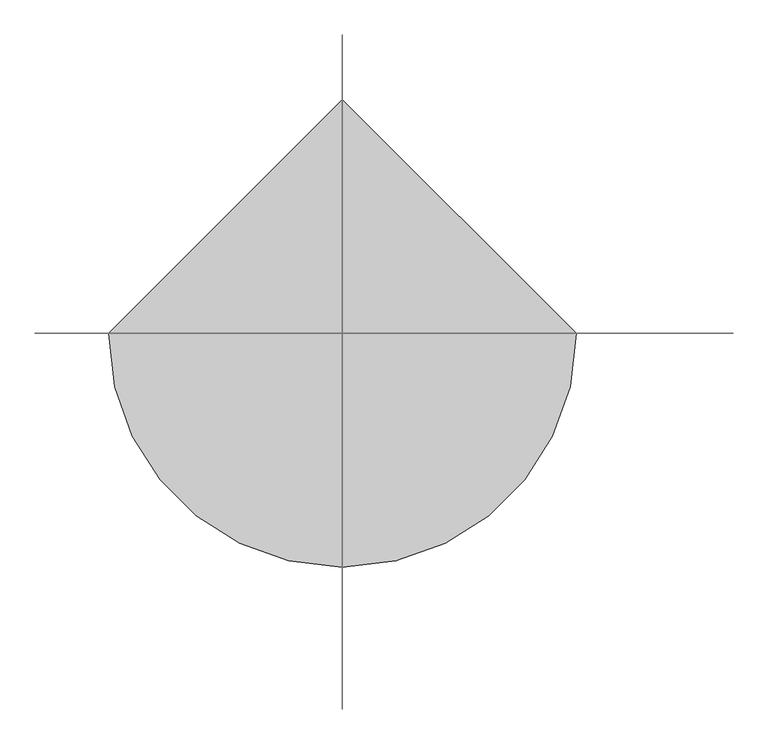
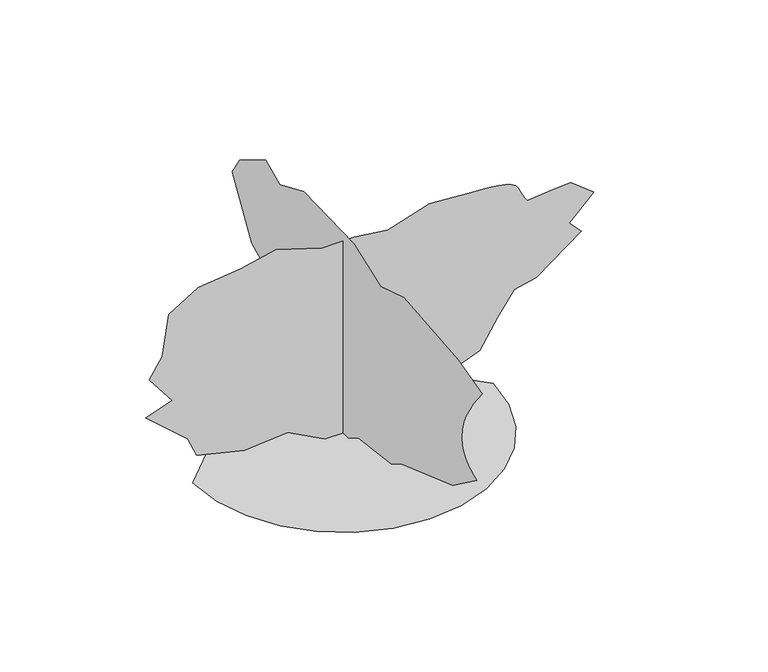
"""IFC4 building model written with IfcOpenShell, lengths in millimetres: proxy geometry, meyer lilac 26082 : meyer lilac 26082."""

from ifc_helpers import new_model, si_unit, origin, place, context, project, spatial, triangles, source, transform, mapped, element, save


def entourage_ea84321d(model_context):
    return source(origin(), model_context, "Body", "Tessellation", [
        triangles([(-84.8149175, 7.75e-05, 8.6e-06), (-258.4957951, 7.39e-05, 93.6967881), (-462.1199759, 8.49e-05, 75.7298434), (-683.7121187, 8.82e-05, 129.6306776), (-725.6373213, 7.86e-05, 225.4544616), (-923.2722055, 6.65e-05, 399.1355936), (-797.5040829, 5.6e-05, 441.0582891), (-905.306805, 4.43e-05, 578.805041), (-845.4161293, 3.03e-05, 674.6290976), (-815.4720268, 5.4e-06, 872.2639091), (-677.7253475, -1.06e-05, 956.1093), (-480.0879198, -2.21e-05, 980.0666313), (-312.397138, -3.37e-05, 1015.9999758), (-96.7927928, -3.53e-05, 950.1199854), (52.9315665, -4.18e-05, 950.1199854), (208.6452405, -4.65e-05, 932.1545849), (406.2806153, -6.23e-05, 992.0452606), (615.896636, -7e-05, 980.0666313), (655.4622442, -7.14e-05, 977.3944834), (693.7171766, -7.27e-05, 974.0950481), (729.355917, -7.37e-05, 969.5382769), (761.0627026, -7.43e-05, 963.0943388), (787.5346333, -7.44e-05, 954.1382721), (807.455801, -7.38e-05, 942.0377026), (819.5208349, -7.25e-05, 926.1652702), (826.871549, -7.08e-05, 909.594334), (833.5949759, -6.94e-05, 895.540468), (839.7925627, -6.83e-05, 883.5796429), (845.5736052, -6.73e-05, 873.2951689), (851.0371525, -6.65e-05, 864.2680309), (856.2924276, -6.57e-05, 856.0790686), (861.443494, -6.5e-05, 848.309194), (975.2355309, -7.14e-05, 860.2852798), (1065.0702364, -7.61e-05, 866.2745945), (1172.8703424, -7.08e-05, 782.4292036), (1059.0809217, -5.23e-05, 668.6397102), (1112.9822828, -4.75e-05, 608.7490708), (903.3662258, -1.97e-05, 453.0343749), (801.5554344, -1.24e-05, 429.0796597), (723.6968147, 3.8e-06, 321.2769739), (639.8513512, 2.39e-05, 183.5315118), (328.4245391, 5.18e-05, 63.7517137), (202.6561802, 5.51e-05, 81.7186584), (100.8435812, 6.93e-05, 5e-07), (0.021362, 58.648346, 1.19e-05), (0.0213578, 202.8161995, 40.9414963), (0.021352, 346.9843074, 46.4863159), (0.021347, 407.9773141, 151.839669), (0.0213581, 335.8946863, 196.1989981), (0.0213523, 457.8832432, 223.9235958), (0.0213509, 607.5959435, 323.7331467), (0.0213526, 563.2348432, 406.9054682), (0.0213517, 740.6741215, 490.0802968), (0.0213453, 895.9316505, 750.6918966), (0.021359, 834.9361004, 844.9538755), (0.0213677, 624.230357, 972.4872248), (0.0213728, 513.3314575, 917.0390104), (0.0213802, 319.2602002, 1000.2113319), (0.0213989, -85.5197618, 989.1216745), (0.0214104, -307.3171429, 911.4942181), (0.0214172, -490.2987428, 966.9424324), (0.021433, -933.8919062, 928.1286678), (0.0214469, -1127.9631998, 878.2227751), (0.0214342, -1091.3973358, 830.7450771), (0.0214336, -1056.4291214, 783.5569691), (0.021433, -1024.6639091, 736.9505116), (0.0214322, -997.699276, 691.2152945), (0.0214311, -977.1354149, 646.6458492), (0.0214298, -964.575135, 603.5319111), (0.0214281, -961.6160133, 562.1629609), (0.0214263, -967.0643726, 525.9679318), (0.0214245, -978.0421909, 497.337085), (0.0214229, -993.625106, 475.0130116), (0.0214213, -1012.893552, 457.7308542), (0.0214197, -1034.9280355, 444.2332769), (0.0214305, -1058.8065926, 433.2554223), (0.021429, -1083.6046429, 423.5399179), (0.0214189, -889.5333492, 279.3720463), (0.0213939, -473.6642567, 135.2049558), (0.021383, -390.489428, 85.3005619), (0.0213686, -124.3337626, 52.0311355), (0.0213699, -41.160192, 0.0), (-701.8553427, 0.0, 8.48e-05), (-683.3005886, -160.8188175, 0.000114), (-630.4584652, -308.5058421, 9.41e-05), (-547.5554223, -438.8281563, 0.0001242), (-438.8281563, -547.5554223, 0.0001065), (-308.5058421, -630.4559217, 9.09e-05), (-160.8188175, -683.3005886, 0.0001273), (3.04e-05, -701.8553427, 0.0001181), (160.8190719, -683.3005886, 0.0001133), (308.5058421, -630.4559217, 0.0001131), (438.8281563, -547.5554223, 0.0001173), (547.5554223, -438.8281563, 0.0001255), (630.4559217, -308.5058421, 8.82e-05), (683.3005886, -160.8188175, 0.0001035), (701.8553427, 6.14e-05, 0.0001219), (-9.28e-05, 701.8553427, 8.86e-05)], [[5, 6, 7], [34, 35, 36], [33, 34, 36], [36, 37, 38], [32, 33, 36], [32, 36, 38], [32, 38, 39], [7, 8, 9], [3, 4, 5], [9, 10, 11], [9, 11, 12], [7, 9, 12], [5, 7, 12], [3, 5, 12], [2, 3, 12], [2, 12, 13], [2, 13, 14], [2, 14, 15], [1, 2, 15], [44, 1, 15], [43, 44, 15], [43, 15, 16], [42, 43, 16], [41, 42, 16], [40, 41, 16], [40, 16, 17], [39, 40, 17], [32, 39, 17], [32, 17, 18], [32, 18, 19], [31, 32, 19], [30, 31, 19], [30, 19, 20], [29, 30, 20], [29, 20, 21], [28, 29, 21], [27, 28, 21], [27, 21, 22], [26, 27, 22], [26, 22, 23], [26, 23, 24], [26, 24, 25], [76, 77, 78], [62, 63, 64], [75, 76, 78], [74, 75, 78], [62, 64, 65], [47, 48, 49], [46, 47, 49], [50, 51, 52], [73, 74, 78], [62, 65, 66], [53, 54, 55], [53, 55, 56], [53, 56, 57], [52, 53, 57], [72, 73, 78], [52, 57, 58], [52, 58, 59], [50, 52, 59], [49, 50, 59], [49, 59, 60], [46, 49, 60], [45, 46, 60], [82, 45, 60], [81, 82, 60], [80, 81, 60], [79, 80, 60], [78, 79, 60], [78, 60, 61], [72, 78, 61], [71, 72, 61], [70, 71, 61], [70, 61, 62], [69, 70, 62], [68, 69, 62], [67, 68, 62], [67, 62, 66], [97, 98, 83], [96, 97, 83], [96, 83, 84], [95, 96, 84], [95, 84, 85], [95, 85, 86], [94, 95, 86], [93, 94, 86], [93, 86, 87], [93, 87, 88], [93, 88, 89], [93, 89, 90], [93, 90, 91], [93, 91, 92]], closed=False),
    ])


if __name__ == "__main__":
    model = new_model("IFC4")
    model_context = context("Model", 3, world=origin())
    ifc_project = project(units=[si_unit("LENGTHUNIT", "METRE", prefix="MILLI")], contexts=[model_context])
    site = spatial("IfcSite", under=ifc_project)
    building = spatial("IfcBuilding", under=site)
    placement = place(None, origin())
    entourage_shape = entourage_ea84321d(model_context)
    element("IfcBuildingElementProxy", 1, Name="meyer lilac 26082 : meyer lilac 26082", ObjectType="meyer lilac 26082 : meyer lilac 26082", at=placement, inside=building, context=model_context, shape_type="MappedRepresentation", body=[
        mapped(entourage_shape, transform((0.0, 0.0, 0.0), x_axis=(1.0, 0.0, 0.0), y_axis=(0.0, 1.0, 0.0), z_axis=(0.0, 0.0, 1.0))),
    ])
    save(model, "model.ifc")

# Revit data of these elements
# Type "meyer lilac 26082 : meyer lilac 26082"
#   built-in parameter 1005195 = "RPC-16-FXGN-2JPX-PG7M-U000-ST1L-LVER-AU"
#   Height = 0
